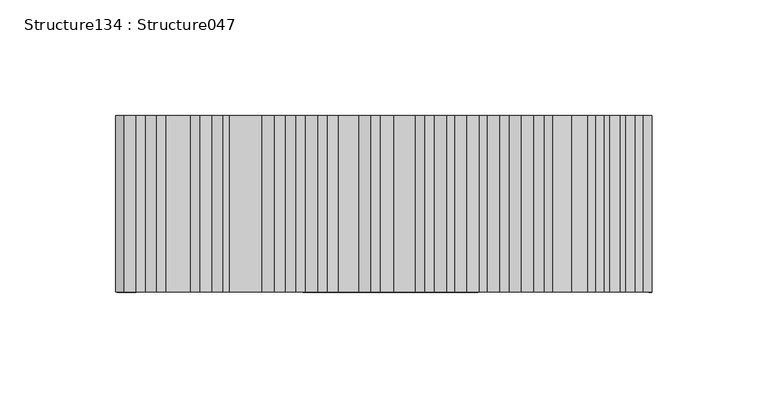
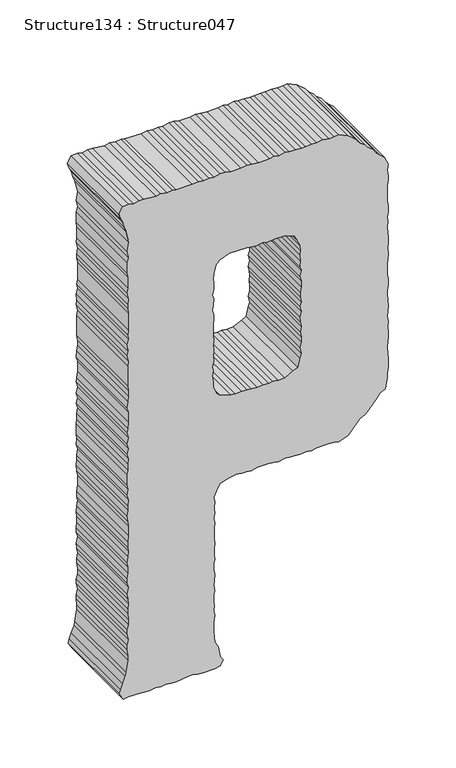
"""IFC4 building model written with IfcOpenShell, lengths in millimetres: proxy geometry, Structure134 : Structure047."""

from ifc_helpers import new_model, si_unit, frame, origin, place, context, project, spatial, polyline, outline, extrude, source, transform, mapped, element, save


def structure134_structure047_4f64f248(model_context):
    return source(origin(), model_context, "Body", "SweptSolid", [
        extrude(outline(polyline([(3996.390138, -46257.2952038), (3996.390138, -46266.0868318), (3997.5486624, -46270.7706723), (3997.5486624, -46274.8800644), (3996.390138, -46280.1463764), (3996.9645864, -46284.2477455), (3996.390138, -46288.939609), (3996.9645864, -46293.6234496), (3996.390138, -46298.8897615), (3996.390138, -46312.9493061), (3996.9645864, -46315.8921508), (3996.390138, -46320.5663636), (3997.5486624, -46325.8503263), (3996.390138, -46329.9516953), (3997.5486624, -46340.4939469), (3997.5486624, -46344.5937114), (3996.390138, -46349.2855749), (3997.5486624, -46353.386944), (3996.9645864, -46358.653256), (3991.6806238, -46362.170549), (3986.4046842, -46360.4215301), (3982.8793681, -46358.653256), (3978.2035506, -46357.4786855), (3973.5197101, -46355.728062), (3962.9774586, -46353.386944), (3954.7506513, -46354.5534915), (3948.917914, -46353.386944), (3944.8165449, -46354.5534915), (3935.4328178, -46354.5534915), (3931.3346579, -46353.9694154), (3921.3748778, -46353.9694154), (3917.2735087, -46354.5534915), (3912.0071968, -46353.386944), (3906.7328618, -46353.9694154), (3903.2059411, -46353.9694154), (3898.5301236, -46353.386944), (3883.2863809, -46353.386944), (3879.1769888, -46353.9694154), (3875.0772243, -46353.386944), (3870.4030114, -46354.5534915), (3864.5446004, -46353.9694154), (3860.4432313, -46354.5534915), (3855.1769193, -46353.386944), (3851.0595042, -46353.9694154), (3832.8921721, -46353.9694154), (3828.2163546, -46353.386944), (3823.5341187, -46353.386944), (3818.8310229, -46353.9694154), (3812.9726119, -46354.5534915), (3808.8888934, -46353.386944), (3800.0876378, -46353.386944), (3794.2292268, -46353.9694154), (3790.7039107, -46354.5534915), (3786.0280932, -46353.386944), (3780.1616592, -46354.5534915), (3776.0618947, -46353.386944), (3771.3860772, -46354.5534915), (3766.684586, -46353.386944), (3762.0023501, -46353.9694154), (3756.7440611, -46353.9694154), (3752.6170184, -46354.5534915), (3743.2332913, -46354.5534915), (3739.1592005, -46353.9694154), (3733.8736333, -46354.5534915), (3729.7738688, -46353.386944), (3723.9154578, -46353.9694154), (3720.4158154, -46353.9694154), (3715.1302482, -46354.5534915), (3709.8559132, -46353.9694154), (3705.7545441, -46353.386944), (3696.9709391, -46353.386944), (3691.0868544, -46353.9694154), (3686.4030139, -46353.9694154), (3682.8857208, -46353.386944), (3678.2018803, -46353.9694154), (3672.9435914, -46354.5534915), (3668.8261762, -46353.9694154), (3662.9854159, -46353.9694154), (3658.3015753, -46354.5534915), (3654.1841602, -46354.5534915), (3650.1004418, -46353.386944), (3644.2420307, -46354.5534915), (3639.5405396, -46353.9694154), (3635.4407751, -46353.386944), (3630.7392839, -46353.9694154), (3626.6571701, -46353.9694154), (3620.7971545, -46353.386944), (3616.0972679, -46353.386944), (3612.0135494, -46354.5534915), (3607.8961343, -46354.5534915), (3602.6298224, -46353.386944), (3597.9540049, -46354.5534915), (3593.8285667, -46354.5534915), (3588.5702778, -46353.9694154), (3584.4689087, -46353.9694154), (3573.9266571, -46355.728062), (3570.4109687, -46356.320161), (3564.54293, -46358.653256), (3559.8671125, -46360.4215301), (3556.3417965, -46361.57845), (3550.4833855, -46358.0707845), (3551.0658569, -46353.9694154), (3551.0658569, -46344.0112399), (3550.4833855, -46340.4939469), (3550.4833855, -46335.8020833), (3551.0658569, -46330.5341668), (3550.4833855, -46325.8503263), (3551.0658569, -46321.7425387), (3550.4833855, -46317.0586982), (3550.4833855, -46312.9493061), (3551.6675836, -46302.4070546), (3551.6675836, -46298.8897615), (3551.0658569, -46294.789997), (3550.4833855, -46289.5220805), (3550.4833855, -46279.5542773), (3551.6675836, -46274.8800644), (3556.3417965, -46272.5293189), (3559.8671125, -46274.8800644), (3569.2524442, -46276.630688), (3575.0851816, -46279.5542773), (3584.4689087, -46280.7304524), (3593.2541183, -46280.7304524), (3599.1125293, -46279.5542773), (3603.7963698, -46280.7304524), (3607.3393366, -46280.1463764), (3613.1720739, -46280.7304524), (3617.8559144, -46280.7304524), (3621.3732075, -46279.5542773), (3626.6571701, -46280.7304524), (3630.7392839, -46280.1463764), (3636.0408972, -46279.5542773), (3640.7167147, -46280.7304524), (3645.9830266, -46280.7304524), (3649.5003197, -46279.5542773), (3654.7842823, -46280.1463764), (3659.4584952, -46280.1463764), (3664.1423357, -46279.5542773), (3668.8261762, -46280.1463764), (3677.6274319, -46280.1463764), (3683.4858429, -46279.5542773), (3687.587212, -46280.7304524), (3691.6869765, -46279.5542773), (3696.3884676, -46280.1463764), (3702.229228, -46279.5542773), (3706.3289925, -46280.7304524), (3713.9556777, -46277.2131594), (3716.8985223, -46274.8800644), (3719.2316172, -46267.2549839), (3720.4158154, -46261.3949683), (3719.8140887, -46256.7031047), (3719.8140887, -46252.6033402), (3719.2316172, -46248.5115988), (3720.4158154, -46243.2356592), (3720.4158154, -46234.4344035), (3719.8140887, -46228.5840155), (3719.2316172, -46225.0667225), (3720.4158154, -46219.7907829), (3719.8140887, -46215.6910184), (3719.8140887, -46209.8326074), (3719.2316172, -46206.3233374), (3719.8140887, -46201.6314738), (3719.2316172, -46196.9396103), (3720.4158154, -46192.2637928), (3720.4158154, -46182.2879666), (3719.8140887, -46177.0216547), (3719.2316172, -46173.5123846), (3722.1568112, -46165.303228), (3726.8566978, -46161.2034636), (3733.8736333, -46155.3354249), (3736.2163558, -46150.661212), (3739.1592005, -46147.7183674), (3747.3587295, -46140.6934089), (3750.8583719, -46138.3506863), (3753.2171405, -46133.6588228), (3762.5848215, -46131.9098039), (3767.2590344, -46131.9098039), (3771.9605256, -46130.7336288), (3780.1616592, -46130.7336288), (3784.8438951, -46131.3177048), (3790.1294623, -46131.9098039), (3795.4037973, -46131.3177048), (3799.5051664, -46130.7336288), (3804.1890069, -46130.7336288), (3808.8888934, -46131.3177048), (3812.9726119, -46130.7336288), (3818.8310229, -46131.9098039), (3822.348316, -46131.3177048), (3827.6162325, -46130.7336288), (3838.1761347, -46131.9098039), (3841.6741725, -46131.9098039), (3846.3772683, -46130.7336288), (3851.6612309, -46130.7336288), (3856.3161885, -46131.9098039), (3865.7015202, -46131.9098039), (3869.8189354, -46131.3177048), (3874.5043805, -46130.7336288), (3880.3627915, -46131.3177048), (3885.0626781, -46130.7336288), (3889.7208449, -46130.7336288), (3893.822214, -46131.3177048), (3899.7046941, -46131.9098039), (3904.3901392, -46131.3177048), (3908.46423, -46131.9098039), (3912.5896682, -46130.7336288), (3918.4480792, -46130.7336288), (3923.1319197, -46131.9098039), (3936.6186205, -46131.9098039), (3941.8753048, -46130.7336288), (3945.4182716, -46130.7336288), (3950.6765605, -46131.9098039), (3955.9348494, -46130.7336288), (3963.5615346, -46134.2493172), (3966.5043792, -46137.7682149), (3970.5768654, -46141.8679794), (3974.1214368, -46144.2107019), (3977.6194746, -46148.8929379), (3980.5623192, -46151.2436835), (3983.4794902, -46154.7609765), (3987.5792547, -46158.2782696), (3994.0233463, -46165.303228), (3997.5486624, -46173.5123846), (3996.9645864, -46177.0216547), (3996.9645864, -46181.7054952), (3997.5486624, -46186.9798302), (3996.9645864, -46192.2637928), (3996.9645864, -46196.3475112), (3996.390138, -46201.6314738), (3996.390138, -46205.1407439), (3996.9645864, -46210.4247065), (3996.9645864, -46215.6910184), (3997.5486624, -46219.2002884), (3996.390138, -46224.4842511), (3997.5486624, -46228.5840155), (3996.390138, -46232.68378), (3996.390138, -46242.0514611), (3996.9645864, -46247.9194997), (3997.5486624, -46252.0272872), (3996.390138, -46257.2952038)]), holes=[polyline([(3797.1463977, -46275.4545129), (3799.5051664, -46277.8052584), (3805.9476534, -46280.7304524), (3810.6298893, -46280.7304524), (3816.4883003, -46281.3129239), (3821.1737455, -46280.7304524), (3824.7167122, -46281.3129239), (3829.9733965, -46280.1463764), (3834.0474873, -46280.7304524), (3839.3587282, -46280.1463764), (3844.6154125, -46280.7304524), (3848.1166595, -46280.1463764), (3853.4198774, -46280.7304524), (3862.8036045, -46280.7304524), (3867.4601667, -46280.1463764), (3871.5599312, -46280.1463764), (3876.263027, -46281.3129239), (3880.3627915, -46280.7304524), (3886.2051565, -46280.1463764), (3889.7208449, -46281.3129239), (3894.4030808, -46280.1463764), (3899.7046941, -46280.1463764), (3904.3901392, -46280.7304524), (3909.0627475, -46280.1463764), (3916.0909152, -46278.3877299), (3919.6066036, -46275.4545129), (3922.5494483, -46266.6709078), (3922.5494483, -46252.0272872), (3921.9733953, -46247.3354237), (3921.3748778, -46243.8181306), (3922.5494483, -46238.5437956), (3921.3748778, -46234.4344035), (3921.9733953, -46228.5840155), (3921.9733953, -46219.2002884), (3919.0321552, -46211.5816263), (3915.5068392, -46209.8326074), (3909.0627475, -46206.9074134), (3904.3901392, -46206.3233374), (3900.2887701, -46206.9074134), (3895.0048075, -46206.3233374), (3889.7208449, -46206.9074134), (3886.2051565, -46205.7328429), (3880.9452629, -46206.9074134), (3876.263027, -46205.7328429), (3870.9790644, -46205.7328429), (3866.3032469, -46206.3233374), (3862.2018778, -46206.3233374), (3857.5019912, -46205.7328429), (3854.0007442, -46206.9074134), (3848.7167816, -46205.7328429), (3844.0345457, -46206.9074134), (3839.3587282, -46206.3233374), (3835.2332901, -46205.7328429), (3830.5574726, -46206.3233374), (3825.849563, -46205.7328429), (3821.1737455, -46205.7328429), (3816.4883003, -46206.9074134), (3810.6298893, -46205.7328429), (3807.1045732, -46206.9074134), (3798.9050443, -46208.6564323), (3797.1463977, -46212.7658244), (3793.6451507, -46219.7907829), (3793.0723069, -46225.0667225), (3793.6451507, -46229.758586), (3793.0723069, -46233.2758791), (3793.6451507, -46237.9516966), (3793.0723069, -46243.2356592), (3793.6451507, -46248.5115988), (3793.6451507, -46252.0272872), (3794.2292268, -46256.7031047), (3793.6451507, -46261.9790443), (3794.2292268, -46266.0868318), (3797.1463977, -46275.4545129)])]), frame((0.0, 247945.1599557, 0.0), z_axis=(0.0, 1.0, 0.0), x_axis=(0.0, 0.0, 1.0)), (0.0, 0.0, 1.0), 76.2),
    ])


if __name__ == "__main__":
    model = new_model("IFC4")
    model_context = context("Model", 3, world=origin())
    ifc_project = project(units=[si_unit("LENGTHUNIT", "METRE", prefix="MILLI")], contexts=[model_context])
    site = spatial("IfcSite", under=ifc_project)
    building = spatial("IfcBuilding", under=site)
    placement = place(None, origin())
    structure134_structure047_shape = structure134_structure047_4f64f248(model_context)
    element("IfcBuildingElementProxy", 1, Name="Structure134 : Structure047", ObjectType="Structure134 : Structure047", at=placement, inside=building, context=model_context, shape_type="MappedRepresentation", body=[
        mapped(structure134_structure047_shape, transform((0.0, 0.0, 0.0), x_axis=(1.0, 0.0, 0.0), y_axis=(0.0, 1.0, 0.0), z_axis=(0.0, 0.0, 1.0))),
    ])
    save(model, "model.ifc")

# Revit data of these elements
# Type "Structure134 : Structure047"
#   NameOverride = "Structure047"
# Element 1 (IfcBuildingElementProxy, "Structure134 : Structure047")
#   Materials on its faces: "BRUSHED ALUM. LETTERING"
# Materials
#   "BRUSHED ALUM. LETTERING": class "Unassigned", colour RGB 169 181 186, transparency 0, Cost = 0
